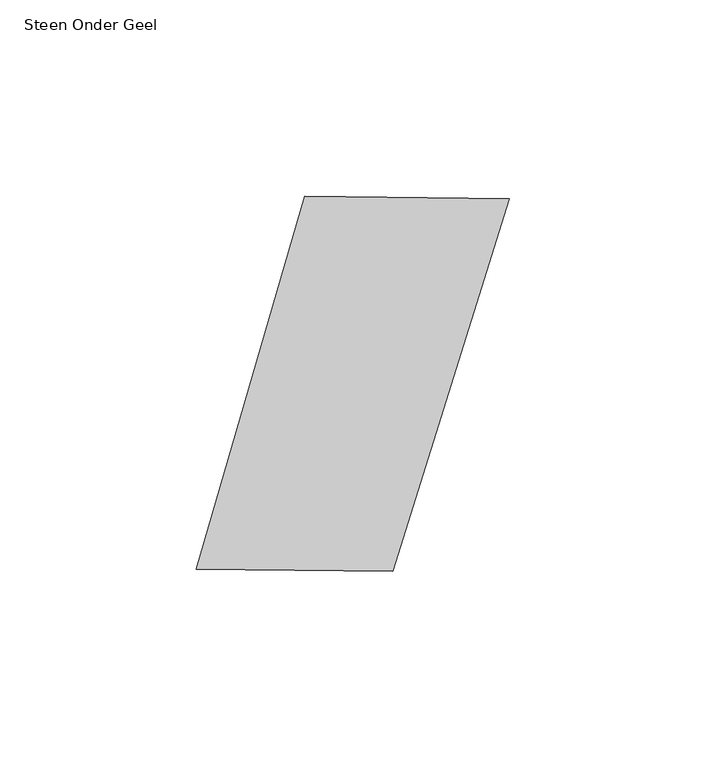
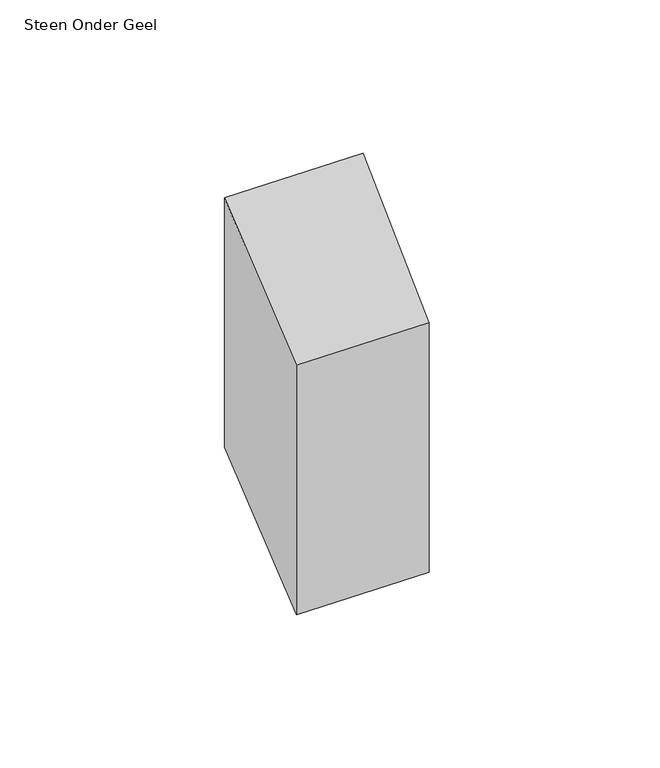
"""IFC4 building model written with IfcOpenShell, lengths in millimetres: proxy geometry, 00_GMA_steen_versie_4 : Steen Onder Geel."""

from ifc_helpers import new_model, si_unit, origin, origin_with_axes, place, context, project, spatial, polyline, outline, extrude, source, transform, mapped, element, save


def steen_onder_geel_0d8976a4(model_context):
    return source(origin(), model_context, "Body", "SweptSolid", [
        extrude(outline(polyline([(114.6454347, 113.7014531), (84.9687392, 18.8340352), (34.9721705, 19.4197989), (62.5250289, 114.288221), (114.6454347, 113.7014531)])), origin_with_axes(), (0.0, 0.0, 1.0), 100.0),
    ])


if __name__ == "__main__":
    model = new_model("IFC4")
    model_context = context("Model", 3, world=origin())
    ifc_project = project(units=[si_unit("LENGTHUNIT", "METRE", prefix="MILLI")], contexts=[model_context])
    site = spatial("IfcSite", under=ifc_project)
    building = spatial("IfcBuilding", under=site)
    placement = place(None, origin())
    steen_onder_geel_shape = steen_onder_geel_0d8976a4(model_context)
    element("IfcBuildingElementProxy", 1, Name="00_GMA_steen_versie_4 : Steen Onder Geel", ObjectType="00_GMA_steen_versie_4 : Steen Onder Geel", at=placement, inside=building, context=model_context, shape_type="MappedRepresentation", body=[
        mapped(steen_onder_geel_shape, transform((0.0, 0.0, 0.0), x_axis=(1.0, 0.0, 0.0), y_axis=(0.0, 1.0, 0.0), z_axis=(0.0, 0.0, 1.0))),
    ])
    save(model, "model.ifc")

# Revit data of these elements
# Type "00_GMA_steen_versie_4 : Steen Onder Geel"
#   StootVoegHalfBoven [instance default] = 5 mm
#   StootVoegHalf [instance default] = 5 mm
#   StootVoegBreedteOnder = 10 mm
#   StootVoegBreedteBoven = 10 mm
#   Steendikte = 100 mm
#   LintVoegOnderHalf = 0 mm
#   LintVoegOnder = 0 mm
#   LintVoegBovenHalf = 5 mm
#   LintVoegBoven = 10 mm
#   materiaal = 21_steen_geel
#   MateriaalVoeg = none
#   Default Elevation = 0
# Element 1 (IfcBuildingElementProxy, "00_GMA_steen_versie_4 : Steen Onder Geel")
#   Materials on its faces: "21_steen_geel"
# Materials
#   "21_steen_geel": class "Unassigned", colour RGB 202 202 0, transparency 0, Cost = 0
